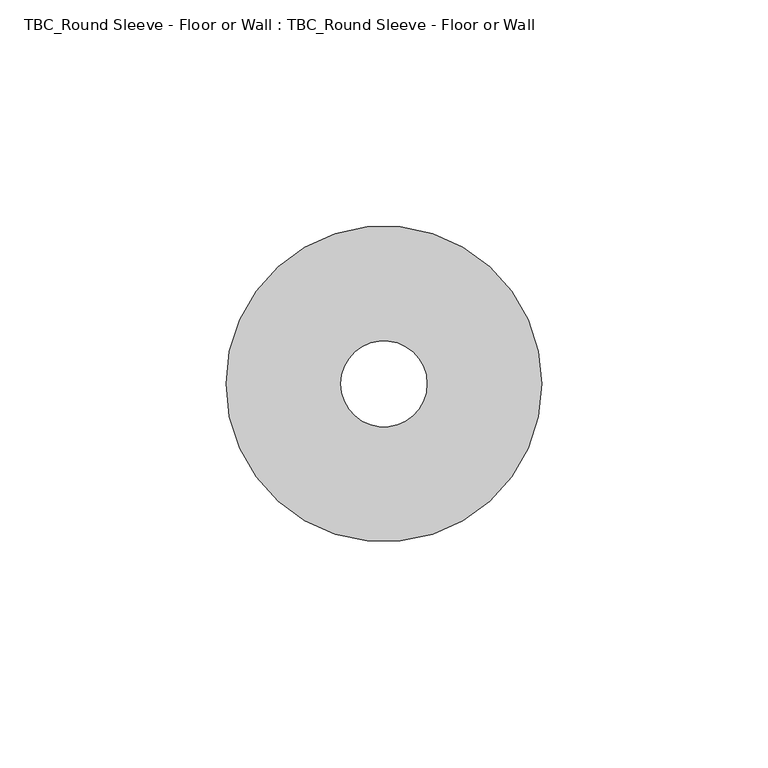
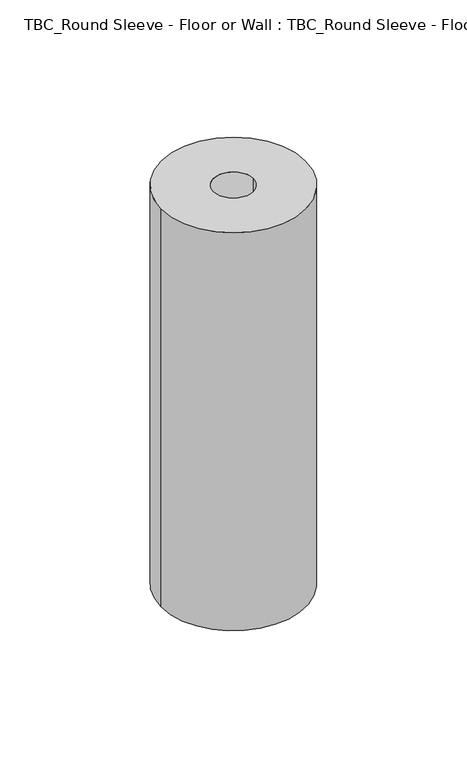
"""IFC4 building model written with IfcOpenShell, lengths in millimetres: proxy geometry, TBC_Round Sleeve - Floor or Wall : TBC_Round Sleeve - Floor or Wall."""

from ifc_helpers import new_model, si_unit, point, frame, origin, origin_2d, place, context, project, spatial, circle_curve, trimmed, segment, composite_curve, outline, extrude, source, transform, mapped, element, save


def tbc_round_sleeve_floor_or_wall_tbc_round_sleeve_floor_or_48347627(model_context):
    return source(origin(), model_context, "Body", "SweptSolid", [
        extrude(outline(composite_curve([segment(trimmed(circle_curve(origin_2d(), 34.925), [point((-34.925, 0.0))], [point((34.925, 0.0))], False, "CARTESIAN"), True, "CONTINUOUS"), segment(trimmed(circle_curve(origin_2d(), 34.925), [point((34.925, 0.0))], [point((-34.925, 0.0))], False, "CARTESIAN"), True, "CONTINUOUS")], self_intersect=False), holes=[composite_curve([segment(trimmed(circle_curve(origin_2d(), 9.525), [point((-9.525, 0.0))], [point((9.525, 0.0))], True, "CARTESIAN"), True, "CONTINUOUS"), segment(trimmed(circle_curve(origin_2d(), 9.525), [point((9.525, 0.0))], [point((-9.525, 0.0))], True, "CARTESIAN"), True, "CONTINUOUS")], self_intersect=False)]), frame((0.0, 0.0, -203.2), z_axis=(0.0, 0.0, 1.0), x_axis=(1.0, 0.0, 0.0)), (0.0, 0.0, 1.0), 203.2),
    ])


if __name__ == "__main__":
    model = new_model("IFC4")
    model_context = context("Model", 3, world=origin())
    ifc_project = project(units=[si_unit("LENGTHUNIT", "METRE", prefix="MILLI")], contexts=[model_context])
    site = spatial("IfcSite", under=ifc_project)
    building = spatial("IfcBuilding", under=site)
    placement = place(None, origin())
    tbc_round_sleeve_floor_or_wall_tbc_round_sleeve_floor_or_shape = tbc_round_sleeve_floor_or_wall_tbc_round_sleeve_floor_or_48347627(model_context)
    element("IfcBuildingElementProxy", 1, Name="TBC_Round Sleeve - Floor or Wall : TBC_Round Sleeve - Floor or Wall", ObjectType="TBC_Round Sleeve - Floor or Wall : TBC_Round Sleeve - Floor or Wall", at=placement, inside=building, context=model_context, shape_type="MappedRepresentation", body=[
        mapped(tbc_round_sleeve_floor_or_wall_tbc_round_sleeve_floor_or_shape, transform((0.0, 0.0, 0.0), x_axis=(1.0, 0.0, 0.0), y_axis=(0.0, 1.0, 0.0), z_axis=(0.0, 0.0, 1.0))),
    ])
    save(model, "model.ifc")

# Revit data of these elements
# Type "TBC_Round Sleeve - Floor or Wall : TBC_Round Sleeve - Floor or Wall"
#   Tag Dimension [instance default] = ""
#   MEP Type [instance default] = ""
#   MEP Element [instance default] = ""
#   MEP Category [instance default] = ""
#   Host Element Type [instance default] = ""
#   Host Element Id [instance default] = ""
#   Host Element Category [instance default] = ""
#   Control Line Y [instance default] = ""
#   Control Line X [instance default] = ""
#   Sleeve Radius [instance default] = 1' - 0"
#   Sleeve Edge [instance default] = 1' - 2"
#   Sleeve Depth [instance default] = 3' - 0"
#   Distance Y [instance default] = 0' - 0"
#   Distance X [instance default] = 0' - 0"
#   Default Elevation = 0
# Element 1 (IfcBuildingElementProxy, "TBC_Round Sleeve - Floor or Wall : TBC_Round Sleeve - Floor or Wall")
#   Tag Dimension = "0.75\"ø"
#   MEP Type = "Mechanical-CWS"
#   MEP Element = "871687"
#   MEP Category = "Pipe"
#   Host Element Type = "8\" Plank"
#   Host Element Id = "732382"
#   Host Element Category = "Floors"
#   Sleeve Radius = 0' - 0 3/4"
#   Sleeve Edge = 0' - 2 3/4"
#   Sleeve Depth = 0' - 8"
